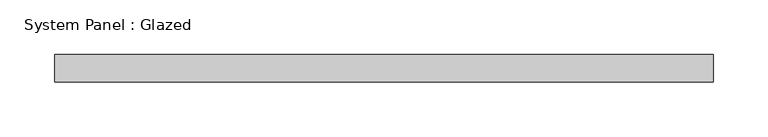
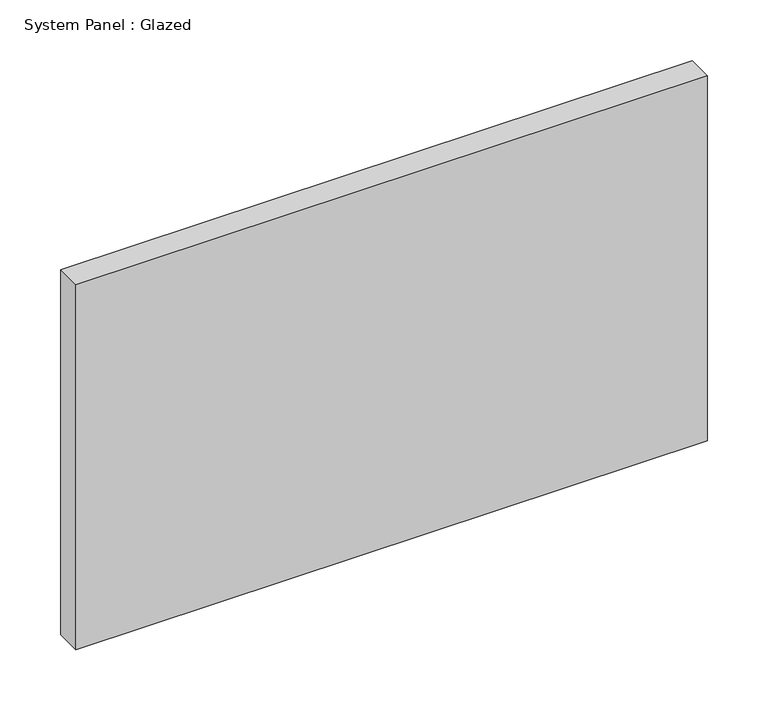
"""IFC4 building model written with IfcOpenShell, lengths in millimetres: plate geometry, System Panel : Glazed."""

from ifc_helpers import new_model, si_unit, origin, origin_with_axes, place, context, project, spatial, polyline, outline, extrude, source, transform, mapped, element, save


def system_panel_glazed_38b4a4ae(model_context):
    return source(origin(), model_context, "Body", "SweptSolid", [
        extrude(outline(polyline([(300.0, 24.5), (-300.0, 24.5), (-300.0, 49.5), (300.0, 49.5), (300.0, 24.5)])), origin_with_axes(), (0.0, 0.0, 1.0), 366.6666667),
    ])


if __name__ == "__main__":
    model = new_model("IFC4")
    model_context = context("Model", 3, world=origin())
    ifc_project = project(units=[si_unit("LENGTHUNIT", "METRE", prefix="MILLI")], contexts=[model_context])
    site = spatial("IfcSite", under=ifc_project)
    building = spatial("IfcBuilding", under=site)
    placement = place(None, origin())
    system_panel_glazed_shape = system_panel_glazed_38b4a4ae(model_context)
    element("IfcPlate", 1, ObjectType="System Panel : Glazed", at=placement, inside=building, context=model_context, shape_type="MappedRepresentation", body=[
        mapped(system_panel_glazed_shape, transform((0.0, 0.0, 0.0), x_axis=(1.0, 0.0, 0.0), y_axis=(0.0, 1.0, 0.0), z_axis=(0.0, 0.0, 1.0))),
    ])
    save(model, "model.ifc")

# Revit data of these elements
# Element 1 (IfcPlate, "System Panel : Glazed")
#   Materials on its faces: "Glass"
# Materials
#   "Glass": class "Glass", colour RGB 218 227 224, transparency 0.85, Description = "Soda Lime Glass", Cost = 0
